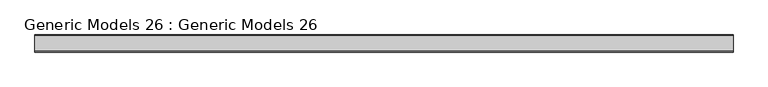
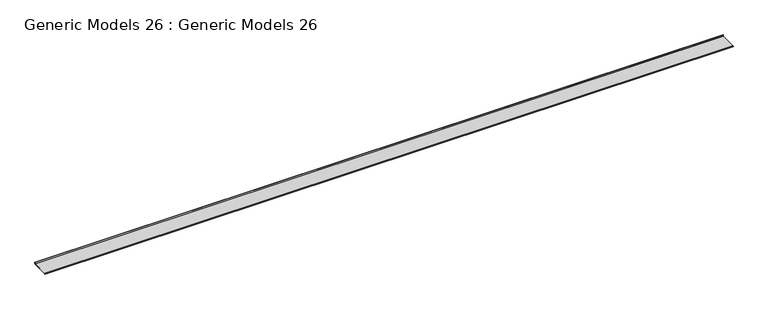
"""IFC4 building model written with IfcOpenShell, lengths in millimetres: proxy geometry, Generic Models 26 : Generic Models 26."""

from ifc_helpers import new_model, si_unit, frame, origin, place, context, project, spatial, polyline, outline, extrude, source, transform, mapped, element, save


def generic_models_26_generic_models_26_b2be200a(model_context):
    return source(origin(), model_context, "Body", "SweptSolid", [
        extrude(outline(polyline([(25634.7777764, 269343.2255146), (25492.6965264, 269343.2255146), (25488.2063983, 269338.7353865), (25487.0838663, 269339.8579186), (25492.0389624, 269344.8130146), (25633.1902764, 269344.8130146), (25633.1902764, 269357.475), (25634.7777764, 269357.475), (25634.7777764, 269343.2255146)])), frame((27760.6090778, 0.0, 0.0), z_axis=(1.0, 0.0, 0.0), x_axis=(0.0, 1.0, 0.0)), (0.0, 0.0, 1.0), 6032.7256636),
    ])


if __name__ == "__main__":
    model = new_model("IFC4")
    model_context = context("Model", 3, world=origin())
    ifc_project = project(units=[si_unit("LENGTHUNIT", "METRE", prefix="MILLI")], contexts=[model_context])
    site = spatial("IfcSite", under=ifc_project)
    building = spatial("IfcBuilding", under=site)
    placement = place(None, origin())
    generic_models_26_generic_models_26_shape = generic_models_26_generic_models_26_b2be200a(model_context)
    element("IfcBuildingElementProxy", 1, Name="Generic Models 26 : Generic Models 26", ObjectType="Generic Models 26 : Generic Models 26", at=placement, inside=building, context=model_context, shape_type="MappedRepresentation", body=[
        mapped(generic_models_26_generic_models_26_shape, transform((0.0, 0.0, 0.0), x_axis=(1.0, 0.0, 0.0), y_axis=(0.0, 1.0, 0.0), z_axis=(0.0, 0.0, 1.0))),
    ])
    save(model, "model.ifc")

# Revit data of these elements
# Element 1 (IfcBuildingElementProxy, "Generic Models 26 : Generic Models 26")
#   Materials on its faces: "GALV. BRAKE METAL - (COLOR: GALV.)"
# Materials
#   "GALV. BRAKE METAL - (COLOR: GALV.)": class "Generic", colour RGB 234 234 234, transparency 0, Cost = 0
